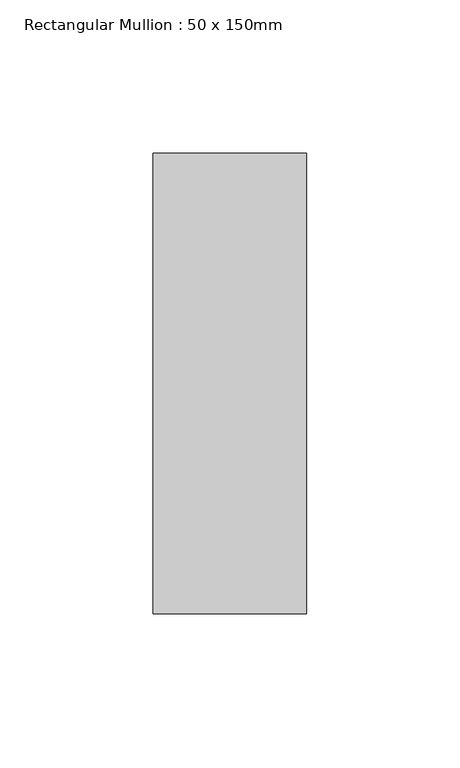
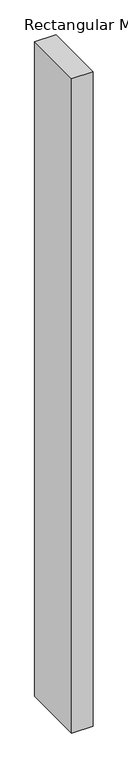
"""IFC4 building model written with IfcOpenShell, lengths in millimetres: member geometry, Rectangular Mullion : 50 x 150mm."""

import ifcopenshell
import ifcopenshell.guid

model = None  # the IFC model being written
_history = None  # IfcOwnerHistory: only IFC2X3 demands one
_inside = {}  # id of a spatial element -> (the spatial element, [elements in it])
_under = {}  # id of a project, library or spatial element -> (it, [spatial elements below it])
_declared = {}  # id of a project -> (the project, [libraries it declares])
_typed = {}  # id of a type object -> (the type object, [elements of that type])
_made_of = {}  # id of a material, layer set ... -> (it, [elements and type objects made of it])


def new_model(schema):
    """Start an empty IFC model of exactly this schema.

    Asked for "IFC4X3", IfcOpenShell would pick the latest addendum, in which some entities
    have other attributes; the version numbers below select the first issue.
    IFC2X3 requires an IfcOwnerHistory on every rooted entity: one is made here for all.
    """
    global model, _history
    if schema == "IFC4X3":
        model = ifcopenshell.file(schema_version=(4, 3, 0, 0))
    else:
        model = ifcopenshell.file(schema=schema)
    _inside.clear()
    _under.clear()
    _declared.clear()
    _typed.clear()
    _made_of.clear()
    _history = None
    if model.schema == "IFC2X3":
        org = make("IfcOrganization", Name="unknown")
        user = make(
            "IfcPersonAndOrganization",
            ThePerson=make("IfcPerson", FamilyName="unknown"),
            TheOrganization=org,
        )
        app = make(
            "IfcApplication",
            ApplicationDeveloper=org,
            Version="unknown",
            ApplicationFullName="unknown",
            ApplicationIdentifier="unknown",
        )
        _history = make(
            "IfcOwnerHistory",
            OwningUser=user,
            OwningApplication=app,
            ChangeAction="ADDED",
            CreationDate=0,
        )
    return model


def make(cls, **values):
    """One entity of the class cls with the attributes given. An attribute that is None is left unset."""
    return model.create_entity(
        cls, **{name: value for name, value in values.items() if value is not None}
    )


def rooted(cls, **values):
    """An entity with a GlobalId (a new one), such as an element, a storey or a relation."""
    return make(cls, GlobalId=ifcopenshell.guid.new(), OwnerHistory=_history, **values)


def si_unit(unit_type, name, prefix=None):
    """IfcSIUnit, for example si_unit("LENGTHUNIT", "METRE", prefix="MILLI")."""
    return make("IfcSIUnit", UnitType=unit_type, Prefix=prefix, Name=name)


def assignment(units):
    """IfcUnitAssignment: the units of a project."""
    return None if units is None else make("IfcUnitAssignment", Units=units)


def point(xyz):
    """IfcCartesianPoint."""
    return None if xyz is None else make("IfcCartesianPoint", Coordinates=xyz)


def direction(xyz):
    """IfcDirection."""
    return None if xyz is None else make("IfcDirection", DirectionRatios=xyz)


def frame(location, z_axis=None, x_axis=None):
    """IfcAxis2Placement3D, a coordinate frame: its origin and axes. An axis left out is left unset."""
    return make(
        "IfcAxis2Placement3D",
        Location=point(location),
        Axis=direction(z_axis),
        RefDirection=direction(x_axis),
    )


def origin():
    """The frame at (0, 0, 0) with its axes left unset."""
    return frame((0.0, 0.0, 0.0))


def place(relative_to, where):
    """IfcLocalPlacement: puts the frame where relative to a parent placement (None: the world)."""
    return make(
        "IfcLocalPlacement", PlacementRelTo=relative_to, RelativePlacement=where
    )


def context(
    kind, dimensions, precision=None, world=None, true_north=None, identifier=None
):
    """IfcGeometricRepresentationContext, for example the 3D "Model" context."""
    return make(
        "IfcGeometricRepresentationContext",
        ContextIdentifier=identifier,
        ContextType=kind,
        CoordinateSpaceDimension=dimensions,
        Precision=precision,
        WorldCoordinateSystem=world,
        TrueNorth=true_north,
    )


def project(units=None, contexts=None):
    """IfcProject with its units and contexts."""
    return rooted(
        "IfcProject",
        Name="project",
        RepresentationContexts=contexts,
        UnitsInContext=assignment(units),
    )


def spatial(cls, under=None, at=None, **own):
    """A site, building, storey or space (cls), placed at a placement, below another one or the project."""
    s = rooted(cls, ObjectPlacement=at, **own)
    if under is not None:
        _under.setdefault(under.id(), (under, []))[1].append(s)
    return s


def polyline(points):
    """IfcPolyline through the points."""
    return make("IfcPolyline", Points=[point(p) for p in points])


def outline(outer, holes=None, kind="AREA"):
    """IfcArbitraryClosedProfileDef: a profile drawn as a closed curve; with holes, ...WithVoids."""
    if holes is None:
        return make("IfcArbitraryClosedProfileDef", ProfileType=kind, OuterCurve=outer)
    return make(
        "IfcArbitraryProfileDefWithVoids",
        ProfileType=kind,
        OuterCurve=outer,
        InnerCurves=holes,
    )


def extrude(swept, where, along, depth):
    """IfcExtrudedAreaSolid: the profile swept, set in the frame where, extruded along a direction by depth."""
    return make(
        "IfcExtrudedAreaSolid",
        SweptArea=swept,
        Position=where,
        ExtrudedDirection=direction(along),
        Depth=depth,
    )


def shape(context_of_items, identifier, shape_type, items):
    """IfcShapeRepresentation: the items that make up one representation, for example the "Body"."""
    return make(
        "IfcShapeRepresentation",
        ContextOfItems=context_of_items,
        RepresentationIdentifier=identifier,
        RepresentationType=shape_type,
        Items=items,
    )


def source(mapping_origin, context_of_items, identifier, shape_type, items):
    """IfcRepresentationMap: a shape defined once, which mapped items show again and again."""
    return make(
        "IfcRepresentationMap",
        MappingOrigin=mapping_origin,
        MappedRepresentation=shape(context_of_items, identifier, shape_type, items),
    )


def transform(
    local_origin,
    x_axis=None,
    y_axis=None,
    z_axis=None,
    scale=None,
    scale2=None,
    scale3=None,
    uniform=True,
):
    """IfcCartesianTransformationOperator3D, or its non-uniform kind. x_axis, y_axis, z_axis: its Axis1, 2, 3."""
    if uniform:
        return make(
            "IfcCartesianTransformationOperator3D",
            Axis1=direction(x_axis),
            Axis2=direction(y_axis),
            LocalOrigin=point(local_origin),
            Scale=scale,
            Axis3=direction(z_axis),
        )
    return make(
        "IfcCartesianTransformationOperator3DnonUniform",
        Axis1=direction(x_axis),
        Axis2=direction(y_axis),
        LocalOrigin=point(local_origin),
        Scale=scale,
        Axis3=direction(z_axis),
        Scale2=scale2,
        Scale3=scale3,
    )


def mapped(mapping_source, mapping_target):
    """IfcMappedItem: shows the shape of a source again, moved by a transform."""
    return make(
        "IfcMappedItem", MappingSource=mapping_source, MappingTarget=mapping_target
    )


def made_of(thing, what):
    """Note that an element or type object is made of a material, layer set ...; save() writes the relation."""
    if what is not None:
        _made_of.setdefault(what.id(), (what, []))[1].append(thing)
    return thing


def element(
    cls,
    number,
    at=None,
    inside=None,
    cuts=None,
    type_object=None,
    material=None,
    context=None,
    identifier="Body",
    shape_type=None,
    held_by="IfcProductDefinitionShape",
    body=None,
    shapes=None,
    **own,
):
    """One element of the class cls, such as IfcWall. Its Tag is "e" and its number.

    at: its placement. inside: the storey or other place that contains it. cuts: it is an
    opening in that element (IfcRelVoidsElement). A single representation is given by context,
    identifier, shape_type and body (its items); several are given by shapes. held_by: the class
    of the entity that holds the representations. save() writes the other relations.
    """
    e = rooted(cls, Tag="e%d" % number, ObjectPlacement=at, **own)
    if body is not None:
        shapes = [shape(context, identifier, shape_type, body)]
    if shapes is not None:
        e.Representation = make(held_by, Representations=shapes)
    if inside is not None:
        _inside.setdefault(inside.id(), (inside, []))[1].append(e)
    if cuts is not None:
        rooted(
            "IfcRelVoidsElement", RelatingBuildingElement=cuts, RelatedOpeningElement=e
        )
    if type_object is not None:
        _typed.setdefault(type_object.id(), (type_object, []))[1].append(e)
    return made_of(e, material)


def aggregate(whole, parts):
    """IfcRelAggregates: a whole, such as a stair, and the parts it consists of."""
    return rooted("IfcRelAggregates", RelatingObject=whole, RelatedObjects=parts)


def save(model, path):
    """Write the relations noted so far, then the file.

    IfcRelAggregates (storeys below a building ...), IfcRelContainedInSpatialStructure (elements
    in a storey), IfcRelDefinesByType, IfcRelAssociatesMaterial and IfcRelDeclares: one each for
    every whole, place, type object, material and project.
    """
    for whole, parts in _under.values():
        aggregate(whole, parts)
    for where, things in _inside.values():
        rooted(
            "IfcRelContainedInSpatialStructure",
            RelatedElements=things,
            RelatingStructure=where,
        )
    for kind, things in _typed.values():
        rooted("IfcRelDefinesByType", RelatedObjects=things, RelatingType=kind)
    for what, things in _made_of.values():
        rooted("IfcRelAssociatesMaterial", RelatedObjects=things, RelatingMaterial=what)
    for by, libraries in _declared.values():
        rooted("IfcRelDeclares", RelatingContext=by, RelatedDefinitions=libraries)
    model.write(path)


def rectangular_mullion_50_x_150mm_128e4daa(model_context):
    return source(origin(), model_context, "Body", "SweptSolid", [
        extrude(outline(polyline([(0.0, 75.0), (0.0, -75.0), (-50.0, -75.0), (-50.0, 75.0), (0.0, 75.0)])), frame((0.0, 0.0, -1615.55), z_axis=(0.0, 0.0, 1.0), x_axis=(1.0, 0.0, 0.0)), (0.0, 0.0, 1.0), 1615.55),
    ])


if __name__ == "__main__":
    model = new_model("IFC4")
    model_context = context("Model", 3, world=origin())
    ifc_project = project(units=[si_unit("LENGTHUNIT", "METRE", prefix="MILLI")], contexts=[model_context])
    site = spatial("IfcSite", under=ifc_project)
    building = spatial("IfcBuilding", under=site)
    placement = place(None, origin())
    rectangular_mullion_50_x_150mm_shape = rectangular_mullion_50_x_150mm_128e4daa(model_context)
    element("IfcMember", 1, ObjectType="Rectangular Mullion : 50 x 150mm", at=placement, inside=building, context=model_context, shape_type="MappedRepresentation", body=[
        mapped(rectangular_mullion_50_x_150mm_shape, transform((0.0, 0.0, 0.0), x_axis=(1.0, 0.0, 0.0), y_axis=(0.0, 1.0, 0.0), z_axis=(0.0, 0.0, 1.0))),
    ])
    save(model, "model.ifc")

# Revit data of these elements
# Type "Rectangular Mullion : 50 x 150mm"
#   Keynote = "H11"
#   built-in parameter 1007304 = 0.492126 (stored number, unit not read)
#   built-in parameter 1007301 = 0.082021 (stored number, unit not read)
#   built-in parameter 1007300 = 0.082021 (stored number, unit not read)
# Element 1 (IfcMember, "Rectangular Mullion : 50 x 150mm")
#   Materials on its faces: "Aluminium"
# Materials
#   "Aluminium": class "Metal", colour RGB 247 247 247, transparency 0, Description = "Aluminium 6061", Cost = 0
